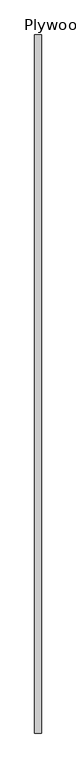
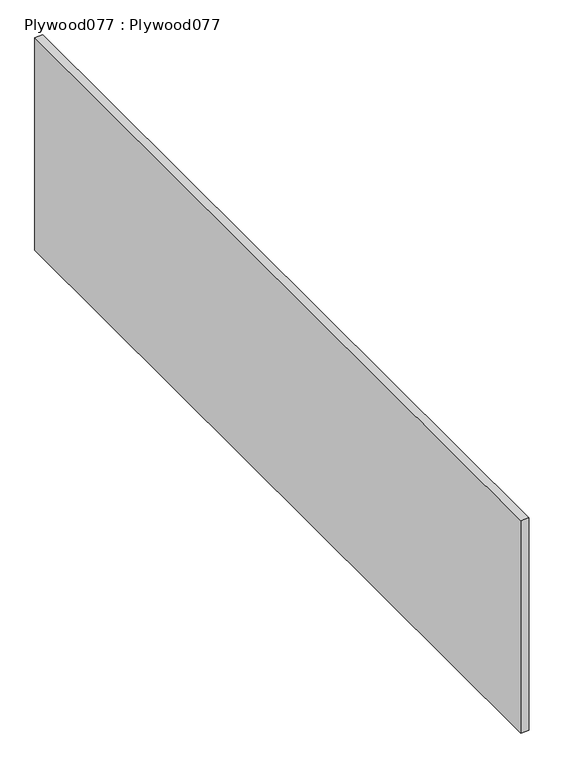
"""IFC4 building model written with IfcOpenShell, lengths in millimetres: proxy geometry, Plywood077 : Plywood077."""

from ifc_helpers import new_model, si_unit, frame, origin, place, context, project, spatial, polyline, outline, extrude, source, transform, mapped, element, save


def plywood077_plywood077_85e516ab(model_context):
    return source(origin(), model_context, "Body", "SweptSolid", [
        extrude(outline(polyline([(-4404.2038825, -1052.8906574), (-4423.2538825, -1052.8906574), (-4423.2538825, 947.1093426), (-4404.2038825, 947.1093426), (-4404.2038825, -1052.8906574)])), frame((0.0, 0.0, 39579.2960083), z_axis=(0.0, 0.0, 1.0), x_axis=(1.0, 0.0, 0.0)), (0.0, 0.0, 1.0), 533.3999917),
    ])


if __name__ == "__main__":
    model = new_model("IFC4")
    model_context = context("Model", 3, world=origin())
    ifc_project = project(units=[si_unit("LENGTHUNIT", "METRE", prefix="MILLI")], contexts=[model_context])
    site = spatial("IfcSite", under=ifc_project)
    building = spatial("IfcBuilding", under=site)
    placement = place(None, origin())
    plywood077_plywood077_shape = plywood077_plywood077_85e516ab(model_context)
    element("IfcBuildingElementProxy", 1, Name="Plywood077 : Plywood077", ObjectType="Plywood077 : Plywood077", at=placement, inside=building, context=model_context, shape_type="MappedRepresentation", body=[
        mapped(plywood077_plywood077_shape, transform((0.0, 0.0, 0.0), x_axis=(1.0, 0.0, 0.0), y_axis=(0.0, 1.0, 0.0), z_axis=(0.0, 0.0, 1.0))),
    ])
    save(model, "model.ifc")

# Revit data of these elements
# Type "Plywood077 : Plywood077"
#   NameOverride = "Plywood077"
# Element 1 (IfcBuildingElementProxy, "Plywood077 : Plywood077")
#   Materials on its faces: "CDX PLYWOOD -  SEE STRUCTURAL DWGS"
# Materials
#   "CDX PLYWOOD -  SEE STRUCTURAL DWGS": class "Unassigned", colour RGB 177 130 114, transparency 0, Cost = 0
